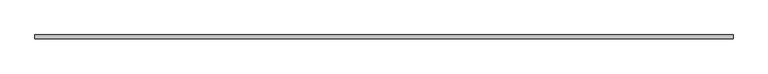
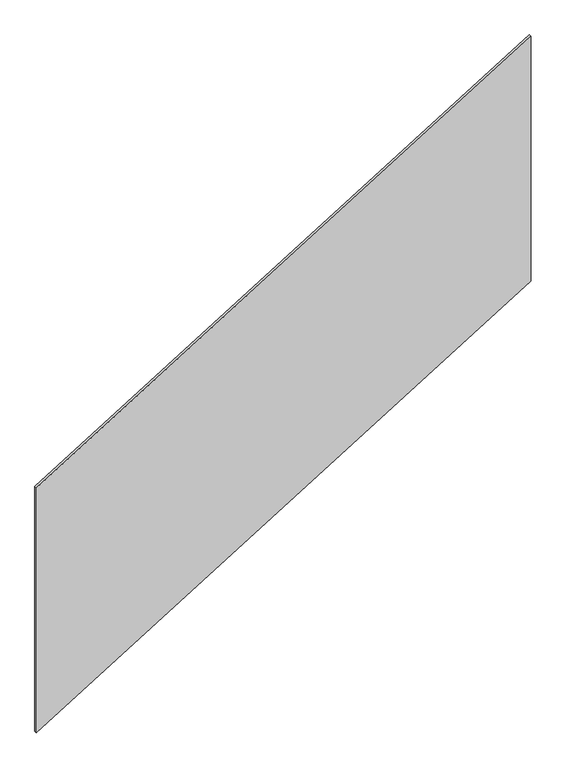
"""IFC4 building model written with IfcOpenShell, lengths in millimetres: railing geometry, ML_Guarda_corpo lance : ML_Guarda_corpo lance."""

import ifcopenshell
import ifcopenshell.guid

model = None  # the IFC model being written
_history = None  # IfcOwnerHistory: only IFC2X3 demands one
_inside = {}  # id of a spatial element -> (the spatial element, [elements in it])
_under = {}  # id of a project, library or spatial element -> (it, [spatial elements below it])
_declared = {}  # id of a project -> (the project, [libraries it declares])
_typed = {}  # id of a type object -> (the type object, [elements of that type])
_made_of = {}  # id of a material, layer set ... -> (it, [elements and type objects made of it])


def new_model(schema):
    """Start an empty IFC model of exactly this schema.

    Asked for "IFC4X3", IfcOpenShell would pick the latest addendum, in which some entities
    have other attributes; the version numbers below select the first issue.
    IFC2X3 requires an IfcOwnerHistory on every rooted entity: one is made here for all.
    """
    global model, _history
    if schema == "IFC4X3":
        model = ifcopenshell.file(schema_version=(4, 3, 0, 0))
    else:
        model = ifcopenshell.file(schema=schema)
    _inside.clear()
    _under.clear()
    _declared.clear()
    _typed.clear()
    _made_of.clear()
    _history = None
    if model.schema == "IFC2X3":
        org = make("IfcOrganization", Name="unknown")
        user = make(
            "IfcPersonAndOrganization",
            ThePerson=make("IfcPerson", FamilyName="unknown"),
            TheOrganization=org,
        )
        app = make(
            "IfcApplication",
            ApplicationDeveloper=org,
            Version="unknown",
            ApplicationFullName="unknown",
            ApplicationIdentifier="unknown",
        )
        _history = make(
            "IfcOwnerHistory",
            OwningUser=user,
            OwningApplication=app,
            ChangeAction="ADDED",
            CreationDate=0,
        )
    return model


def make(cls, **values):
    """One entity of the class cls with the attributes given. An attribute that is None is left unset."""
    return model.create_entity(
        cls, **{name: value for name, value in values.items() if value is not None}
    )


def rooted(cls, **values):
    """An entity with a GlobalId (a new one), such as an element, a storey or a relation."""
    return make(cls, GlobalId=ifcopenshell.guid.new(), OwnerHistory=_history, **values)


def si_unit(unit_type, name, prefix=None):
    """IfcSIUnit, for example si_unit("LENGTHUNIT", "METRE", prefix="MILLI")."""
    return make("IfcSIUnit", UnitType=unit_type, Prefix=prefix, Name=name)


def assignment(units):
    """IfcUnitAssignment: the units of a project."""
    return None if units is None else make("IfcUnitAssignment", Units=units)


def point(xyz):
    """IfcCartesianPoint."""
    return None if xyz is None else make("IfcCartesianPoint", Coordinates=xyz)


def direction(xyz):
    """IfcDirection."""
    return None if xyz is None else make("IfcDirection", DirectionRatios=xyz)


def frame(location, z_axis=None, x_axis=None):
    """IfcAxis2Placement3D, a coordinate frame: its origin and axes. An axis left out is left unset."""
    return make(
        "IfcAxis2Placement3D",
        Location=point(location),
        Axis=direction(z_axis),
        RefDirection=direction(x_axis),
    )


def origin():
    """The frame at (0, 0, 0) with its axes left unset."""
    return frame((0.0, 0.0, 0.0))


def place(relative_to, where):
    """IfcLocalPlacement: puts the frame where relative to a parent placement (None: the world)."""
    return make(
        "IfcLocalPlacement", PlacementRelTo=relative_to, RelativePlacement=where
    )


def context(
    kind, dimensions, precision=None, world=None, true_north=None, identifier=None
):
    """IfcGeometricRepresentationContext, for example the 3D "Model" context."""
    return make(
        "IfcGeometricRepresentationContext",
        ContextIdentifier=identifier,
        ContextType=kind,
        CoordinateSpaceDimension=dimensions,
        Precision=precision,
        WorldCoordinateSystem=world,
        TrueNorth=true_north,
    )


def project(units=None, contexts=None):
    """IfcProject with its units and contexts."""
    return rooted(
        "IfcProject",
        Name="project",
        RepresentationContexts=contexts,
        UnitsInContext=assignment(units),
    )


def spatial(cls, under=None, at=None, **own):
    """A site, building, storey or space (cls), placed at a placement, below another one or the project."""
    s = rooted(cls, ObjectPlacement=at, **own)
    if under is not None:
        _under.setdefault(under.id(), (under, []))[1].append(s)
    return s


def polyline(points):
    """IfcPolyline through the points."""
    return make("IfcPolyline", Points=[point(p) for p in points])


def outline(outer, holes=None, kind="AREA"):
    """IfcArbitraryClosedProfileDef: a profile drawn as a closed curve; with holes, ...WithVoids."""
    if holes is None:
        return make("IfcArbitraryClosedProfileDef", ProfileType=kind, OuterCurve=outer)
    return make(
        "IfcArbitraryProfileDefWithVoids",
        ProfileType=kind,
        OuterCurve=outer,
        InnerCurves=holes,
    )


def extrude(swept, where, along, depth):
    """IfcExtrudedAreaSolid: the profile swept, set in the frame where, extruded along a direction by depth."""
    return make(
        "IfcExtrudedAreaSolid",
        SweptArea=swept,
        Position=where,
        ExtrudedDirection=direction(along),
        Depth=depth,
    )


def shape(context_of_items, identifier, shape_type, items):
    """IfcShapeRepresentation: the items that make up one representation, for example the "Body"."""
    return make(
        "IfcShapeRepresentation",
        ContextOfItems=context_of_items,
        RepresentationIdentifier=identifier,
        RepresentationType=shape_type,
        Items=items,
    )


def source(mapping_origin, context_of_items, identifier, shape_type, items):
    """IfcRepresentationMap: a shape defined once, which mapped items show again and again."""
    return make(
        "IfcRepresentationMap",
        MappingOrigin=mapping_origin,
        MappedRepresentation=shape(context_of_items, identifier, shape_type, items),
    )


def transform(
    local_origin,
    x_axis=None,
    y_axis=None,
    z_axis=None,
    scale=None,
    scale2=None,
    scale3=None,
    uniform=True,
):
    """IfcCartesianTransformationOperator3D, or its non-uniform kind. x_axis, y_axis, z_axis: its Axis1, 2, 3."""
    if uniform:
        return make(
            "IfcCartesianTransformationOperator3D",
            Axis1=direction(x_axis),
            Axis2=direction(y_axis),
            LocalOrigin=point(local_origin),
            Scale=scale,
            Axis3=direction(z_axis),
        )
    return make(
        "IfcCartesianTransformationOperator3DnonUniform",
        Axis1=direction(x_axis),
        Axis2=direction(y_axis),
        LocalOrigin=point(local_origin),
        Scale=scale,
        Axis3=direction(z_axis),
        Scale2=scale2,
        Scale3=scale3,
    )


def mapped(mapping_source, mapping_target):
    """IfcMappedItem: shows the shape of a source again, moved by a transform."""
    return make(
        "IfcMappedItem", MappingSource=mapping_source, MappingTarget=mapping_target
    )


def made_of(thing, what):
    """Note that an element or type object is made of a material, layer set ...; save() writes the relation."""
    if what is not None:
        _made_of.setdefault(what.id(), (what, []))[1].append(thing)
    return thing


def element(
    cls,
    number,
    at=None,
    inside=None,
    cuts=None,
    type_object=None,
    material=None,
    context=None,
    identifier="Body",
    shape_type=None,
    held_by="IfcProductDefinitionShape",
    body=None,
    shapes=None,
    **own,
):
    """One element of the class cls, such as IfcWall. Its Tag is "e" and its number.

    at: its placement. inside: the storey or other place that contains it. cuts: it is an
    opening in that element (IfcRelVoidsElement). A single representation is given by context,
    identifier, shape_type and body (its items); several are given by shapes. held_by: the class
    of the entity that holds the representations. save() writes the other relations.
    """
    e = rooted(cls, Tag="e%d" % number, ObjectPlacement=at, **own)
    if body is not None:
        shapes = [shape(context, identifier, shape_type, body)]
    if shapes is not None:
        e.Representation = make(held_by, Representations=shapes)
    if inside is not None:
        _inside.setdefault(inside.id(), (inside, []))[1].append(e)
    if cuts is not None:
        rooted(
            "IfcRelVoidsElement", RelatingBuildingElement=cuts, RelatedOpeningElement=e
        )
    if type_object is not None:
        _typed.setdefault(type_object.id(), (type_object, []))[1].append(e)
    return made_of(e, material)


def aggregate(whole, parts):
    """IfcRelAggregates: a whole, such as a stair, and the parts it consists of."""
    return rooted("IfcRelAggregates", RelatingObject=whole, RelatedObjects=parts)


def save(model, path):
    """Write the relations noted so far, then the file.

    IfcRelAggregates (storeys below a building ...), IfcRelContainedInSpatialStructure (elements
    in a storey), IfcRelDefinesByType, IfcRelAssociatesMaterial and IfcRelDeclares: one each for
    every whole, place, type object, material and project.
    """
    for whole, parts in _under.values():
        aggregate(whole, parts)
    for where, things in _inside.values():
        rooted(
            "IfcRelContainedInSpatialStructure",
            RelatedElements=things,
            RelatingStructure=where,
        )
    for kind, things in _typed.values():
        rooted("IfcRelDefinesByType", RelatedObjects=things, RelatingType=kind)
    for what, things in _made_of.values():
        rooted("IfcRelAssociatesMaterial", RelatedObjects=things, RelatingMaterial=what)
    for by, libraries in _declared.values():
        rooted("IfcRelDeclares", RelatingContext=by, RelatedDefinitions=libraries)
    model.write(path)


def railing_c44cfcee(model_context):
    return source(origin(), model_context, "Body", "SweptSolid", [
        extrude(outline(polyline([(1672.2222222, -4460.281307), (500.0, -4460.281307), (1877.7777778, -2220.281307), (3050.0, -2220.281307), (1672.2222222, -4460.281307)])), frame((0.0, -5573.3699847, 0.0), z_axis=(0.0, 1.0, 0.0), x_axis=(0.0, 0.0, 1.0)), (0.0, 0.0, 1.0), 12.0),
    ])


if __name__ == "__main__":
    model = new_model("IFC4")
    model_context = context("Model", 3, world=origin())
    ifc_project = project(units=[si_unit("LENGTHUNIT", "METRE", prefix="MILLI")], contexts=[model_context])
    site = spatial("IfcSite", under=ifc_project)
    building = spatial("IfcBuilding", under=site)
    placement = place(None, origin())
    railing_shape = railing_c44cfcee(model_context)
    element("IfcRailing", 1, ObjectType="ML_Guarda_corpo lance : ML_Guarda_corpo lance", at=placement, inside=building, context=model_context, shape_type="MappedRepresentation", body=[
        mapped(railing_shape, transform((0.0, 0.0, 0.0), x_axis=(1.0, 0.0, 0.0), y_axis=(0.0, 1.0, 0.0), z_axis=(0.0, 0.0, 1.0))),
    ])
    save(model, "model.ifc")

# Revit data of these elements
# Type "ML_Guarda_corpo lance : ML_Guarda_corpo lance"
#   ME_Área = 2.62578 m²
#   ME_Espessura [instance default] = 0.012 m
#   ME_Compr Painéis = 2.629804 m
#   ME_Altura = 0.998469 m
#   ME_Material Tipo Vidro [instance default] = .VIDRO GENÉRICO
# Element 1 (IfcRailing, "ML_Guarda_corpo lance : ML_Guarda_corpo lance")
#   Materials on its faces: ".VIDRO GENÉRICO"
# Materials
#   ".VIDRO GENÉRICO": class ".CC_VIDRO", colour RGB 0 128 192, transparency 0.9, Description = "Vidro comum", Cost = 0
